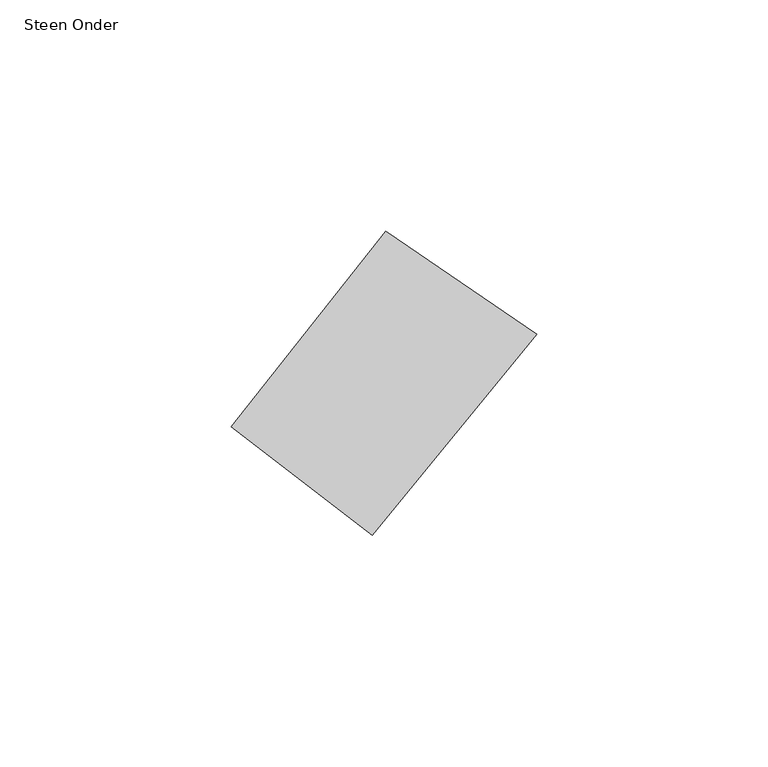
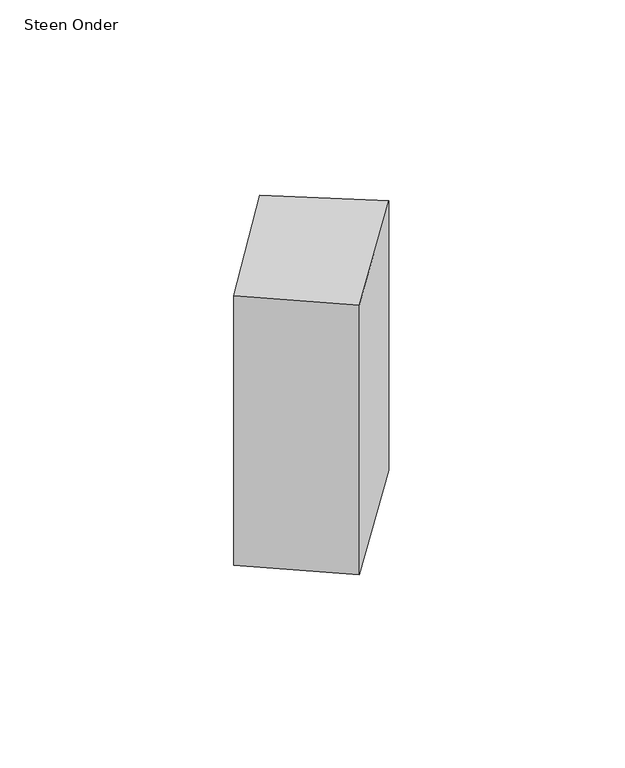
"""IFC4 building model written with IfcOpenShell, lengths in millimetres: proxy geometry, 00_GMA_steen_versie_4 : Steen Onder."""

from ifc_helpers import new_model, si_unit, frame, origin, place, context, project, spatial, polyline, outline, extrude, source, transform, mapped, element, save


def steen_onder_fe9ab8c4(model_context):
    return source(origin(), model_context, "Body", "SweptSolid", [
        extrude(outline(polyline([(116.7657494, 54.8940381), (81.3047621, 11.5494664), (50.8791029, 34.9706965), (84.2154548, 77.1154096), (116.7657494, 54.8940381)])), frame((0.0, 0.0, -100.0), z_axis=(0.0, 0.0, 1.0), x_axis=(1.0, 0.0, 0.0)), (0.0, 0.0, 1.0), 100.0),
    ])


if __name__ == "__main__":
    model = new_model("IFC4")
    model_context = context("Model", 3, world=origin())
    ifc_project = project(units=[si_unit("LENGTHUNIT", "METRE", prefix="MILLI")], contexts=[model_context])
    site = spatial("IfcSite", under=ifc_project)
    building = spatial("IfcBuilding", under=site)
    placement = place(None, origin())
    steen_onder_shape = steen_onder_fe9ab8c4(model_context)
    element("IfcBuildingElementProxy", 1, Name="00_GMA_steen_versie_4 : Steen Onder", ObjectType="00_GMA_steen_versie_4 : Steen Onder", at=placement, inside=building, context=model_context, shape_type="MappedRepresentation", body=[
        mapped(steen_onder_shape, transform((0.0, 0.0, 0.0), x_axis=(1.0, 0.0, 0.0), y_axis=(0.0, 1.0, 0.0), z_axis=(0.0, 0.0, 1.0))),
    ])
    save(model, "model.ifc")

# Revit data of these elements
# Type "00_GMA_steen_versie_4 : Steen Onder"
#   StootVoegHalfBoven [instance default] = 5 mm
#   StootVoegHalf [instance default] = 5 mm
#   StootVoegBreedteOnder = 10 mm
#   StootVoegBreedteBoven = 10 mm
#   Steendikte = 100 mm
#   LintVoegOnderHalf = 0 mm
#   LintVoegOnder = 0 mm
#   LintVoegBovenHalf = 5 mm
#   LintVoegBoven = 10 mm
#   materiaal = none
#   MateriaalVoeg = none
#   Default Elevation = 0
